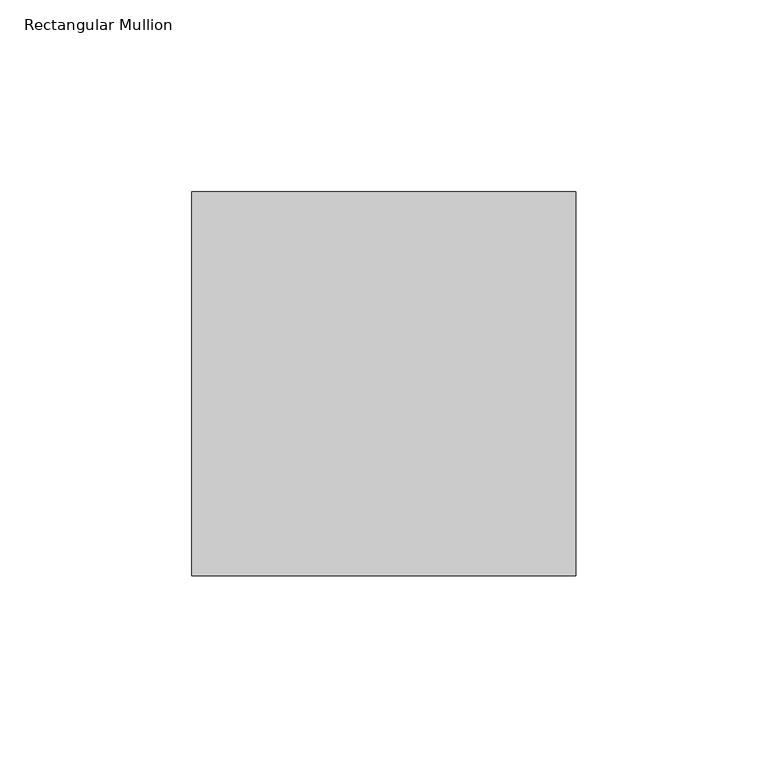
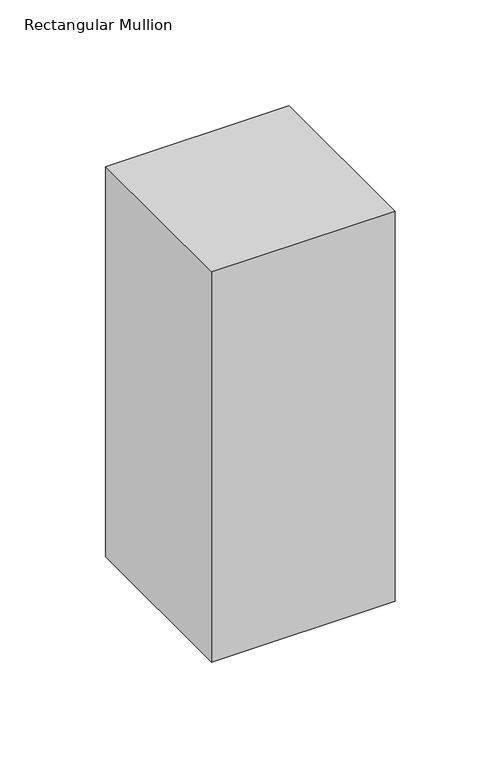
"""IFC4 building model written with IfcOpenShell, lengths in millimetres: member geometry, Rectangular Mullion : 알루미늄_Rectangular Cap_100 x100."""

import ifcopenshell
import ifcopenshell.guid

model = None  # the IFC model being written
_history = None  # IfcOwnerHistory: only IFC2X3 demands one
_inside = {}  # id of a spatial element -> (the spatial element, [elements in it])
_under = {}  # id of a project, library or spatial element -> (it, [spatial elements below it])
_declared = {}  # id of a project -> (the project, [libraries it declares])
_typed = {}  # id of a type object -> (the type object, [elements of that type])
_made_of = {}  # id of a material, layer set ... -> (it, [elements and type objects made of it])


def new_model(schema):
    """Start an empty IFC model of exactly this schema.

    Asked for "IFC4X3", IfcOpenShell would pick the latest addendum, in which some entities
    have other attributes; the version numbers below select the first issue.
    IFC2X3 requires an IfcOwnerHistory on every rooted entity: one is made here for all.
    """
    global model, _history
    if schema == "IFC4X3":
        model = ifcopenshell.file(schema_version=(4, 3, 0, 0))
    else:
        model = ifcopenshell.file(schema=schema)
    _inside.clear()
    _under.clear()
    _declared.clear()
    _typed.clear()
    _made_of.clear()
    _history = None
    if model.schema == "IFC2X3":
        org = make("IfcOrganization", Name="unknown")
        user = make(
            "IfcPersonAndOrganization",
            ThePerson=make("IfcPerson", FamilyName="unknown"),
            TheOrganization=org,
        )
        app = make(
            "IfcApplication",
            ApplicationDeveloper=org,
            Version="unknown",
            ApplicationFullName="unknown",
            ApplicationIdentifier="unknown",
        )
        _history = make(
            "IfcOwnerHistory",
            OwningUser=user,
            OwningApplication=app,
            ChangeAction="ADDED",
            CreationDate=0,
        )
    return model


def make(cls, **values):
    """One entity of the class cls with the attributes given. An attribute that is None is left unset."""
    return model.create_entity(
        cls, **{name: value for name, value in values.items() if value is not None}
    )


def rooted(cls, **values):
    """An entity with a GlobalId (a new one), such as an element, a storey or a relation."""
    return make(cls, GlobalId=ifcopenshell.guid.new(), OwnerHistory=_history, **values)


def si_unit(unit_type, name, prefix=None):
    """IfcSIUnit, for example si_unit("LENGTHUNIT", "METRE", prefix="MILLI")."""
    return make("IfcSIUnit", UnitType=unit_type, Prefix=prefix, Name=name)


def assignment(units):
    """IfcUnitAssignment: the units of a project."""
    return None if units is None else make("IfcUnitAssignment", Units=units)


def point(xyz):
    """IfcCartesianPoint."""
    return None if xyz is None else make("IfcCartesianPoint", Coordinates=xyz)


def direction(xyz):
    """IfcDirection."""
    return None if xyz is None else make("IfcDirection", DirectionRatios=xyz)


def frame(location, z_axis=None, x_axis=None):
    """IfcAxis2Placement3D, a coordinate frame: its origin and axes. An axis left out is left unset."""
    return make(
        "IfcAxis2Placement3D",
        Location=point(location),
        Axis=direction(z_axis),
        RefDirection=direction(x_axis),
    )


def origin():
    """The frame at (0, 0, 0) with its axes left unset."""
    return frame((0.0, 0.0, 0.0))


def place(relative_to, where):
    """IfcLocalPlacement: puts the frame where relative to a parent placement (None: the world)."""
    return make(
        "IfcLocalPlacement", PlacementRelTo=relative_to, RelativePlacement=where
    )


def context(
    kind, dimensions, precision=None, world=None, true_north=None, identifier=None
):
    """IfcGeometricRepresentationContext, for example the 3D "Model" context."""
    return make(
        "IfcGeometricRepresentationContext",
        ContextIdentifier=identifier,
        ContextType=kind,
        CoordinateSpaceDimension=dimensions,
        Precision=precision,
        WorldCoordinateSystem=world,
        TrueNorth=true_north,
    )


def project(units=None, contexts=None):
    """IfcProject with its units and contexts."""
    return rooted(
        "IfcProject",
        Name="project",
        RepresentationContexts=contexts,
        UnitsInContext=assignment(units),
    )


def spatial(cls, under=None, at=None, **own):
    """A site, building, storey or space (cls), placed at a placement, below another one or the project."""
    s = rooted(cls, ObjectPlacement=at, **own)
    if under is not None:
        _under.setdefault(under.id(), (under, []))[1].append(s)
    return s


def polyline(points):
    """IfcPolyline through the points."""
    return make("IfcPolyline", Points=[point(p) for p in points])


def outline(outer, holes=None, kind="AREA"):
    """IfcArbitraryClosedProfileDef: a profile drawn as a closed curve; with holes, ...WithVoids."""
    if holes is None:
        return make("IfcArbitraryClosedProfileDef", ProfileType=kind, OuterCurve=outer)
    return make(
        "IfcArbitraryProfileDefWithVoids",
        ProfileType=kind,
        OuterCurve=outer,
        InnerCurves=holes,
    )


def extrude(swept, where, along, depth):
    """IfcExtrudedAreaSolid: the profile swept, set in the frame where, extruded along a direction by depth."""
    return make(
        "IfcExtrudedAreaSolid",
        SweptArea=swept,
        Position=where,
        ExtrudedDirection=direction(along),
        Depth=depth,
    )


def shape(context_of_items, identifier, shape_type, items):
    """IfcShapeRepresentation: the items that make up one representation, for example the "Body"."""
    return make(
        "IfcShapeRepresentation",
        ContextOfItems=context_of_items,
        RepresentationIdentifier=identifier,
        RepresentationType=shape_type,
        Items=items,
    )


def source(mapping_origin, context_of_items, identifier, shape_type, items):
    """IfcRepresentationMap: a shape defined once, which mapped items show again and again."""
    return make(
        "IfcRepresentationMap",
        MappingOrigin=mapping_origin,
        MappedRepresentation=shape(context_of_items, identifier, shape_type, items),
    )


def transform(
    local_origin,
    x_axis=None,
    y_axis=None,
    z_axis=None,
    scale=None,
    scale2=None,
    scale3=None,
    uniform=True,
):
    """IfcCartesianTransformationOperator3D, or its non-uniform kind. x_axis, y_axis, z_axis: its Axis1, 2, 3."""
    if uniform:
        return make(
            "IfcCartesianTransformationOperator3D",
            Axis1=direction(x_axis),
            Axis2=direction(y_axis),
            LocalOrigin=point(local_origin),
            Scale=scale,
            Axis3=direction(z_axis),
        )
    return make(
        "IfcCartesianTransformationOperator3DnonUniform",
        Axis1=direction(x_axis),
        Axis2=direction(y_axis),
        LocalOrigin=point(local_origin),
        Scale=scale,
        Axis3=direction(z_axis),
        Scale2=scale2,
        Scale3=scale3,
    )


def mapped(mapping_source, mapping_target):
    """IfcMappedItem: shows the shape of a source again, moved by a transform."""
    return make(
        "IfcMappedItem", MappingSource=mapping_source, MappingTarget=mapping_target
    )


def made_of(thing, what):
    """Note that an element or type object is made of a material, layer set ...; save() writes the relation."""
    if what is not None:
        _made_of.setdefault(what.id(), (what, []))[1].append(thing)
    return thing


def element(
    cls,
    number,
    at=None,
    inside=None,
    cuts=None,
    type_object=None,
    material=None,
    context=None,
    identifier="Body",
    shape_type=None,
    held_by="IfcProductDefinitionShape",
    body=None,
    shapes=None,
    **own,
):
    """One element of the class cls, such as IfcWall. Its Tag is "e" and its number.

    at: its placement. inside: the storey or other place that contains it. cuts: it is an
    opening in that element (IfcRelVoidsElement). A single representation is given by context,
    identifier, shape_type and body (its items); several are given by shapes. held_by: the class
    of the entity that holds the representations. save() writes the other relations.
    """
    e = rooted(cls, Tag="e%d" % number, ObjectPlacement=at, **own)
    if body is not None:
        shapes = [shape(context, identifier, shape_type, body)]
    if shapes is not None:
        e.Representation = make(held_by, Representations=shapes)
    if inside is not None:
        _inside.setdefault(inside.id(), (inside, []))[1].append(e)
    if cuts is not None:
        rooted(
            "IfcRelVoidsElement", RelatingBuildingElement=cuts, RelatedOpeningElement=e
        )
    if type_object is not None:
        _typed.setdefault(type_object.id(), (type_object, []))[1].append(e)
    return made_of(e, material)


def aggregate(whole, parts):
    """IfcRelAggregates: a whole, such as a stair, and the parts it consists of."""
    return rooted("IfcRelAggregates", RelatingObject=whole, RelatedObjects=parts)


def save(model, path):
    """Write the relations noted so far, then the file.

    IfcRelAggregates (storeys below a building ...), IfcRelContainedInSpatialStructure (elements
    in a storey), IfcRelDefinesByType, IfcRelAssociatesMaterial and IfcRelDeclares: one each for
    every whole, place, type object, material and project.
    """
    for whole, parts in _under.values():
        aggregate(whole, parts)
    for where, things in _inside.values():
        rooted(
            "IfcRelContainedInSpatialStructure",
            RelatedElements=things,
            RelatingStructure=where,
        )
    for kind, things in _typed.values():
        rooted("IfcRelDefinesByType", RelatedObjects=things, RelatingType=kind)
    for what, things in _made_of.values():
        rooted("IfcRelAssociatesMaterial", RelatedObjects=things, RelatingMaterial=what)
    for by, libraries in _declared.values():
        rooted("IfcRelDeclares", RelatingContext=by, RelatedDefinitions=libraries)
    model.write(path)


def rectangular_mullion_f7ac6ae7(model_context):
    return source(origin(), model_context, "Body", "SweptSolid", [
        extrude(outline(polyline([(0.0, 50.0), (0.0, -50.0), (-100.0, -50.0), (-100.0, 50.0), (0.0, 50.0)])), frame((0.0, 0.0, -225.0), z_axis=(0.0, 0.0, 1.0), x_axis=(1.0, 0.0, 0.0)), (0.0, 0.0, 1.0), 225.0),
    ])


if __name__ == "__main__":
    model = new_model("IFC4")
    model_context = context("Model", 3, world=origin())
    ifc_project = project(units=[si_unit("LENGTHUNIT", "METRE", prefix="MILLI")], contexts=[model_context])
    site = spatial("IfcSite", under=ifc_project)
    building = spatial("IfcBuilding", under=site)
    placement = place(None, origin())
    rectangular_mullion_shape = rectangular_mullion_f7ac6ae7(model_context)
    element("IfcMember", 1, ObjectType="Rectangular Mullion : 알루미늄_Rectangular Cap_100 x100", at=placement, inside=building, context=model_context, shape_type="MappedRepresentation", body=[
        mapped(rectangular_mullion_shape, transform((0.0, 0.0, 0.0), x_axis=(1.0, 0.0, 0.0), y_axis=(0.0, 1.0, 0.0), z_axis=(0.0, 0.0, 1.0))),
    ])
    save(model, "model.ifc")

# Revit data of these elements
# Type "Rectangular Mullion : 알루미늄_Rectangular Cap_100 x100"
#   built-in parameter 1007304 = 0.328084 (stored number, unit not read)
#   built-in parameter 1007301 = 0.164042 (stored number, unit not read)
#   built-in parameter 1007300 = 0.164042 (stored number, unit not read)
# Element 1 (IfcMember, "Rectangular Mullion : 알루미늄_Rectangular Cap_100 x100")
#   Materials on its faces: "00_Metal_Stainless Steel"
# Materials
#   "00_Metal_Stainless Steel": class "Metal", colour RGB 148 148 148, transparency 0, Description = "Steel", Cost = 0
